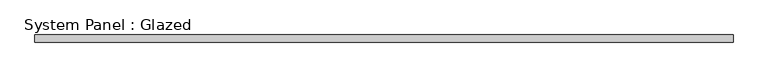
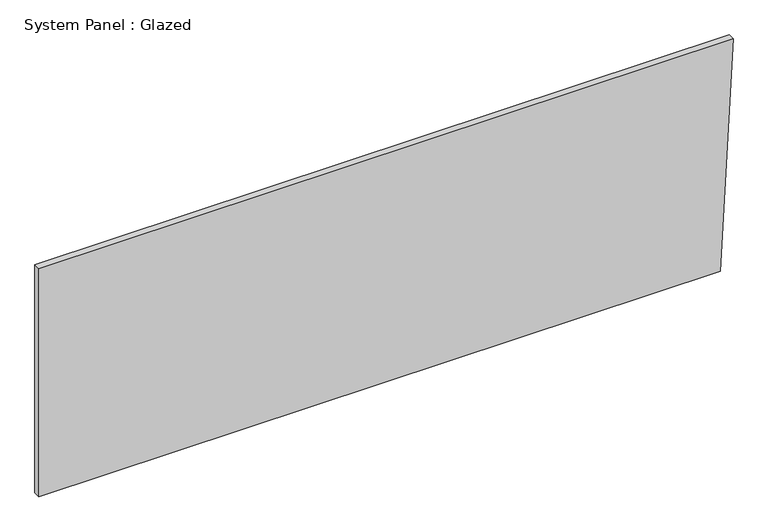
"""IFC4 building model written with IfcOpenShell, lengths in millimetres: plate geometry, System Panel : Glazed."""

import ifcopenshell
import ifcopenshell.guid

model = None  # the IFC model being written
_history = None  # IfcOwnerHistory: only IFC2X3 demands one
_inside = {}  # id of a spatial element -> (the spatial element, [elements in it])
_under = {}  # id of a project, library or spatial element -> (it, [spatial elements below it])
_declared = {}  # id of a project -> (the project, [libraries it declares])
_typed = {}  # id of a type object -> (the type object, [elements of that type])
_made_of = {}  # id of a material, layer set ... -> (it, [elements and type objects made of it])


def new_model(schema):
    """Start an empty IFC model of exactly this schema.

    Asked for "IFC4X3", IfcOpenShell would pick the latest addendum, in which some entities
    have other attributes; the version numbers below select the first issue.
    IFC2X3 requires an IfcOwnerHistory on every rooted entity: one is made here for all.
    """
    global model, _history
    if schema == "IFC4X3":
        model = ifcopenshell.file(schema_version=(4, 3, 0, 0))
    else:
        model = ifcopenshell.file(schema=schema)
    _inside.clear()
    _under.clear()
    _declared.clear()
    _typed.clear()
    _made_of.clear()
    _history = None
    if model.schema == "IFC2X3":
        org = make("IfcOrganization", Name="unknown")
        user = make(
            "IfcPersonAndOrganization",
            ThePerson=make("IfcPerson", FamilyName="unknown"),
            TheOrganization=org,
        )
        app = make(
            "IfcApplication",
            ApplicationDeveloper=org,
            Version="unknown",
            ApplicationFullName="unknown",
            ApplicationIdentifier="unknown",
        )
        _history = make(
            "IfcOwnerHistory",
            OwningUser=user,
            OwningApplication=app,
            ChangeAction="ADDED",
            CreationDate=0,
        )
    return model


def make(cls, **values):
    """One entity of the class cls with the attributes given. An attribute that is None is left unset."""
    return model.create_entity(
        cls, **{name: value for name, value in values.items() if value is not None}
    )


def rooted(cls, **values):
    """An entity with a GlobalId (a new one), such as an element, a storey or a relation."""
    return make(cls, GlobalId=ifcopenshell.guid.new(), OwnerHistory=_history, **values)


def si_unit(unit_type, name, prefix=None):
    """IfcSIUnit, for example si_unit("LENGTHUNIT", "METRE", prefix="MILLI")."""
    return make("IfcSIUnit", UnitType=unit_type, Prefix=prefix, Name=name)


def assignment(units):
    """IfcUnitAssignment: the units of a project."""
    return None if units is None else make("IfcUnitAssignment", Units=units)


def point(xyz):
    """IfcCartesianPoint."""
    return None if xyz is None else make("IfcCartesianPoint", Coordinates=xyz)


def direction(xyz):
    """IfcDirection."""
    return None if xyz is None else make("IfcDirection", DirectionRatios=xyz)


def frame(location, z_axis=None, x_axis=None):
    """IfcAxis2Placement3D, a coordinate frame: its origin and axes. An axis left out is left unset."""
    return make(
        "IfcAxis2Placement3D",
        Location=point(location),
        Axis=direction(z_axis),
        RefDirection=direction(x_axis),
    )


def origin():
    """The frame at (0, 0, 0) with its axes left unset."""
    return frame((0.0, 0.0, 0.0))


def place(relative_to, where):
    """IfcLocalPlacement: puts the frame where relative to a parent placement (None: the world)."""
    return make(
        "IfcLocalPlacement", PlacementRelTo=relative_to, RelativePlacement=where
    )


def context(
    kind, dimensions, precision=None, world=None, true_north=None, identifier=None
):
    """IfcGeometricRepresentationContext, for example the 3D "Model" context."""
    return make(
        "IfcGeometricRepresentationContext",
        ContextIdentifier=identifier,
        ContextType=kind,
        CoordinateSpaceDimension=dimensions,
        Precision=precision,
        WorldCoordinateSystem=world,
        TrueNorth=true_north,
    )


def project(units=None, contexts=None):
    """IfcProject with its units and contexts."""
    return rooted(
        "IfcProject",
        Name="project",
        RepresentationContexts=contexts,
        UnitsInContext=assignment(units),
    )


def spatial(cls, under=None, at=None, **own):
    """A site, building, storey or space (cls), placed at a placement, below another one or the project."""
    s = rooted(cls, ObjectPlacement=at, **own)
    if under is not None:
        _under.setdefault(under.id(), (under, []))[1].append(s)
    return s


def polyline(points):
    """IfcPolyline through the points."""
    return make("IfcPolyline", Points=[point(p) for p in points])


def outline(outer, holes=None, kind="AREA"):
    """IfcArbitraryClosedProfileDef: a profile drawn as a closed curve; with holes, ...WithVoids."""
    if holes is None:
        return make("IfcArbitraryClosedProfileDef", ProfileType=kind, OuterCurve=outer)
    return make(
        "IfcArbitraryProfileDefWithVoids",
        ProfileType=kind,
        OuterCurve=outer,
        InnerCurves=holes,
    )


def extrude(swept, where, along, depth):
    """IfcExtrudedAreaSolid: the profile swept, set in the frame where, extruded along a direction by depth."""
    return make(
        "IfcExtrudedAreaSolid",
        SweptArea=swept,
        Position=where,
        ExtrudedDirection=direction(along),
        Depth=depth,
    )


def shape(context_of_items, identifier, shape_type, items):
    """IfcShapeRepresentation: the items that make up one representation, for example the "Body"."""
    return make(
        "IfcShapeRepresentation",
        ContextOfItems=context_of_items,
        RepresentationIdentifier=identifier,
        RepresentationType=shape_type,
        Items=items,
    )


def source(mapping_origin, context_of_items, identifier, shape_type, items):
    """IfcRepresentationMap: a shape defined once, which mapped items show again and again."""
    return make(
        "IfcRepresentationMap",
        MappingOrigin=mapping_origin,
        MappedRepresentation=shape(context_of_items, identifier, shape_type, items),
    )


def transform(
    local_origin,
    x_axis=None,
    y_axis=None,
    z_axis=None,
    scale=None,
    scale2=None,
    scale3=None,
    uniform=True,
):
    """IfcCartesianTransformationOperator3D, or its non-uniform kind. x_axis, y_axis, z_axis: its Axis1, 2, 3."""
    if uniform:
        return make(
            "IfcCartesianTransformationOperator3D",
            Axis1=direction(x_axis),
            Axis2=direction(y_axis),
            LocalOrigin=point(local_origin),
            Scale=scale,
            Axis3=direction(z_axis),
        )
    return make(
        "IfcCartesianTransformationOperator3DnonUniform",
        Axis1=direction(x_axis),
        Axis2=direction(y_axis),
        LocalOrigin=point(local_origin),
        Scale=scale,
        Axis3=direction(z_axis),
        Scale2=scale2,
        Scale3=scale3,
    )


def mapped(mapping_source, mapping_target):
    """IfcMappedItem: shows the shape of a source again, moved by a transform."""
    return make(
        "IfcMappedItem", MappingSource=mapping_source, MappingTarget=mapping_target
    )


def made_of(thing, what):
    """Note that an element or type object is made of a material, layer set ...; save() writes the relation."""
    if what is not None:
        _made_of.setdefault(what.id(), (what, []))[1].append(thing)
    return thing


def element(
    cls,
    number,
    at=None,
    inside=None,
    cuts=None,
    type_object=None,
    material=None,
    context=None,
    identifier="Body",
    shape_type=None,
    held_by="IfcProductDefinitionShape",
    body=None,
    shapes=None,
    **own,
):
    """One element of the class cls, such as IfcWall. Its Tag is "e" and its number.

    at: its placement. inside: the storey or other place that contains it. cuts: it is an
    opening in that element (IfcRelVoidsElement). A single representation is given by context,
    identifier, shape_type and body (its items); several are given by shapes. held_by: the class
    of the entity that holds the representations. save() writes the other relations.
    """
    e = rooted(cls, Tag="e%d" % number, ObjectPlacement=at, **own)
    if body is not None:
        shapes = [shape(context, identifier, shape_type, body)]
    if shapes is not None:
        e.Representation = make(held_by, Representations=shapes)
    if inside is not None:
        _inside.setdefault(inside.id(), (inside, []))[1].append(e)
    if cuts is not None:
        rooted(
            "IfcRelVoidsElement", RelatingBuildingElement=cuts, RelatedOpeningElement=e
        )
    if type_object is not None:
        _typed.setdefault(type_object.id(), (type_object, []))[1].append(e)
    return made_of(e, material)


def aggregate(whole, parts):
    """IfcRelAggregates: a whole, such as a stair, and the parts it consists of."""
    return rooted("IfcRelAggregates", RelatingObject=whole, RelatedObjects=parts)


def save(model, path):
    """Write the relations noted so far, then the file.

    IfcRelAggregates (storeys below a building ...), IfcRelContainedInSpatialStructure (elements
    in a storey), IfcRelDefinesByType, IfcRelAssociatesMaterial and IfcRelDeclares: one each for
    every whole, place, type object, material and project.
    """
    for whole, parts in _under.values():
        aggregate(whole, parts)
    for where, things in _inside.values():
        rooted(
            "IfcRelContainedInSpatialStructure",
            RelatedElements=things,
            RelatingStructure=where,
        )
    for kind, things in _typed.values():
        rooted("IfcRelDefinesByType", RelatedObjects=things, RelatingType=kind)
    for what, things in _made_of.values():
        rooted("IfcRelAssociatesMaterial", RelatedObjects=things, RelatingMaterial=what)
    for by, libraries in _declared.values():
        rooted("IfcRelDeclares", RelatingContext=by, RelatedDefinitions=libraries)
    model.write(path)


def system_panel_glazed_a884192e(model_context):
    return source(origin(), model_context, "Body", "SweptSolid", [
        extrude(outline(polyline([(0.0, -1247.3520184), (0.0, 1202.0248119), (866.081558, 1247.3520184), (866.081558, -1247.3520184), (0.0, -1247.3520184)])), frame((0.0, -44.45, 0.0), z_axis=(0.0, 1.0, 0.0), x_axis=(0.0, 0.0, 1.0)), (0.0, 0.0, 1.0), 25.4),
    ])


if __name__ == "__main__":
    model = new_model("IFC4")
    model_context = context("Model", 3, world=origin())
    ifc_project = project(units=[si_unit("LENGTHUNIT", "METRE", prefix="MILLI")], contexts=[model_context])
    site = spatial("IfcSite", under=ifc_project)
    building = spatial("IfcBuilding", under=site)
    placement = place(None, origin())
    system_panel_glazed_shape = system_panel_glazed_a884192e(model_context)
    element("IfcPlate", 1, ObjectType="System Panel : Glazed", at=placement, inside=building, context=model_context, shape_type="MappedRepresentation", body=[
        mapped(system_panel_glazed_shape, transform((0.0, 0.0, 0.0), x_axis=(1.0, 0.0, 0.0), y_axis=(0.0, 1.0, 0.0), z_axis=(0.0, 0.0, 1.0))),
    ])
    save(model, "model.ifc")

# Revit data of these elements
# Type "System Panel : Glazed"
#   Construction Type Id = "GSP4R"
#   Analytic Construction = "1/8 in Pilkington single glazing"
#   Visual Light Transmittance = 0.9
#   Solar Heat Gain Coefficient = 0.86
#   Heat Transfer Coefficient (U) = 1.18115 BTU/(h·ft²·°F)
#   Define Thermal Properties by = 1
# Element 1 (IfcPlate, "System Panel : Glazed")
#   Materials on its faces: "Glass"
# Materials
#   "Glass": class "Glass", colour RGB 0 128 192, transparency 0.75, Description = "Soda Lime Glass", Cost = 0
